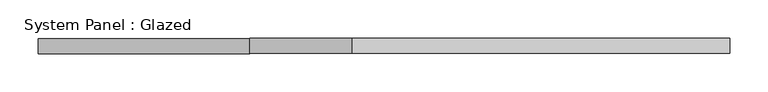
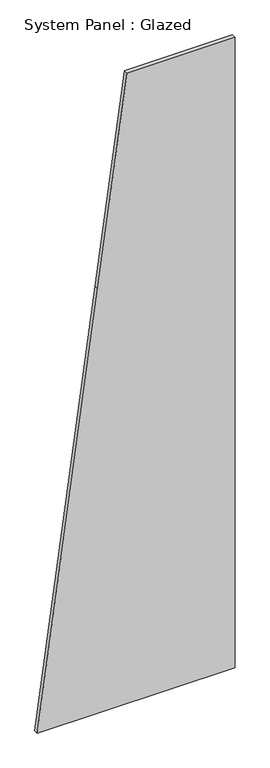
"""IFC4 building model written with IfcOpenShell, lengths in millimetres: plate geometry, System Panel : Glazed."""

from ifc_helpers import new_model, si_unit, frame, origin, place, context, project, spatial, polyline, outline, extrude, source, transform, mapped, element, save


def system_panel_glazed_b2cff3bf(model_context):
    return source(origin(), model_context, "Body", "SweptSolid", [
        extrude(outline(polyline([(0.0, -453.2663), (0.0, 453.2663), (2060.0, 453.2663), (3050.0, 453.2663), (3050.0, -41.5085337), (2053.3105573, -176.0641464), (0.0, -453.2663)])), frame((0.0, 0.0, 0.0), z_axis=(0.0, 1.0, 0.0), x_axis=(0.0, 0.0, 1.0)), (0.0, 0.0, 1.0), 20.0),
    ])


if __name__ == "__main__":
    model = new_model("IFC4")
    model_context = context("Model", 3, world=origin())
    ifc_project = project(units=[si_unit("LENGTHUNIT", "METRE", prefix="MILLI")], contexts=[model_context])
    site = spatial("IfcSite", under=ifc_project)
    building = spatial("IfcBuilding", under=site)
    placement = place(None, origin())
    system_panel_glazed_shape = system_panel_glazed_b2cff3bf(model_context)
    element("IfcPlate", 1, ObjectType="System Panel : Glazed", at=placement, inside=building, context=model_context, shape_type="MappedRepresentation", body=[
        mapped(system_panel_glazed_shape, transform((0.0, 0.0, 0.0), x_axis=(1.0, 0.0, 0.0), y_axis=(0.0, 1.0, 0.0), z_axis=(0.0, 0.0, 1.0))),
    ])
    save(model, "model.ifc")

# Revit data of these elements
# Type "System Panel : Glazed"
#   COBie.Type = no
# Element 1 (IfcPlate, "System Panel : Glazed")
#   Materials on its faces: "Glass"
# Materials
#   "Glass": class "Glass", colour RGB 0 128 192, transparency 0.75, Description = "Soda Lime Glass", Cost = 0
